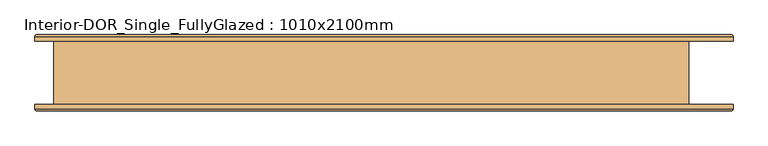
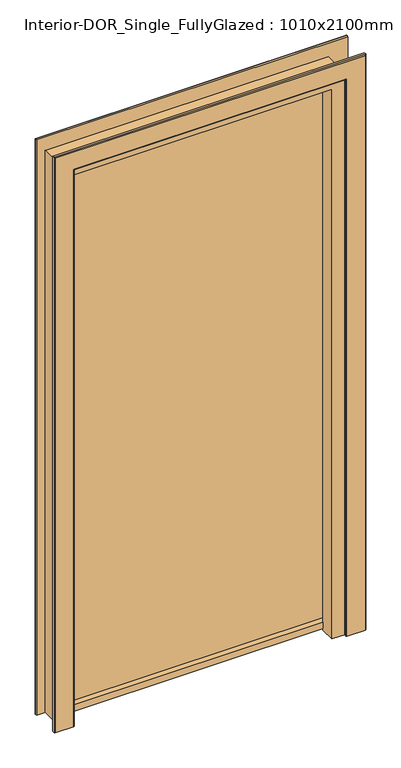
"""IFC4 building model written with IfcOpenShell, lengths in millimetres: door geometry, Interior-DOR_Single_FullyGlazed : 1010x2100mm."""

import ifcopenshell
import ifcopenshell.guid

model = None  # the IFC model being written
_history = None  # IfcOwnerHistory: only IFC2X3 demands one
_inside = {}  # id of a spatial element -> (the spatial element, [elements in it])
_under = {}  # id of a project, library or spatial element -> (it, [spatial elements below it])
_declared = {}  # id of a project -> (the project, [libraries it declares])
_typed = {}  # id of a type object -> (the type object, [elements of that type])
_made_of = {}  # id of a material, layer set ... -> (it, [elements and type objects made of it])


def new_model(schema):
    """Start an empty IFC model of exactly this schema.

    Asked for "IFC4X3", IfcOpenShell would pick the latest addendum, in which some entities
    have other attributes; the version numbers below select the first issue.
    IFC2X3 requires an IfcOwnerHistory on every rooted entity: one is made here for all.
    """
    global model, _history
    if schema == "IFC4X3":
        model = ifcopenshell.file(schema_version=(4, 3, 0, 0))
    else:
        model = ifcopenshell.file(schema=schema)
    _inside.clear()
    _under.clear()
    _declared.clear()
    _typed.clear()
    _made_of.clear()
    _history = None
    if model.schema == "IFC2X3":
        org = make("IfcOrganization", Name="unknown")
        user = make(
            "IfcPersonAndOrganization",
            ThePerson=make("IfcPerson", FamilyName="unknown"),
            TheOrganization=org,
        )
        app = make(
            "IfcApplication",
            ApplicationDeveloper=org,
            Version="unknown",
            ApplicationFullName="unknown",
            ApplicationIdentifier="unknown",
        )
        _history = make(
            "IfcOwnerHistory",
            OwningUser=user,
            OwningApplication=app,
            ChangeAction="ADDED",
            CreationDate=0,
        )
    return model


def make(cls, **values):
    """One entity of the class cls with the attributes given. An attribute that is None is left unset."""
    return model.create_entity(
        cls, **{name: value for name, value in values.items() if value is not None}
    )


def rooted(cls, **values):
    """An entity with a GlobalId (a new one), such as an element, a storey or a relation."""
    return make(cls, GlobalId=ifcopenshell.guid.new(), OwnerHistory=_history, **values)


def si_unit(unit_type, name, prefix=None):
    """IfcSIUnit, for example si_unit("LENGTHUNIT", "METRE", prefix="MILLI")."""
    return make("IfcSIUnit", UnitType=unit_type, Prefix=prefix, Name=name)


def assignment(units):
    """IfcUnitAssignment: the units of a project."""
    return None if units is None else make("IfcUnitAssignment", Units=units)


def point(xyz):
    """IfcCartesianPoint."""
    return None if xyz is None else make("IfcCartesianPoint", Coordinates=xyz)


def direction(xyz):
    """IfcDirection."""
    return None if xyz is None else make("IfcDirection", DirectionRatios=xyz)


def frame(location, z_axis=None, x_axis=None):
    """IfcAxis2Placement3D, a coordinate frame: its origin and axes. An axis left out is left unset."""
    return make(
        "IfcAxis2Placement3D",
        Location=point(location),
        Axis=direction(z_axis),
        RefDirection=direction(x_axis),
    )


def origin():
    """The frame at (0, 0, 0) with its axes left unset."""
    return frame((0.0, 0.0, 0.0))


def place(relative_to, where):
    """IfcLocalPlacement: puts the frame where relative to a parent placement (None: the world)."""
    return make(
        "IfcLocalPlacement", PlacementRelTo=relative_to, RelativePlacement=where
    )


def context(
    kind, dimensions, precision=None, world=None, true_north=None, identifier=None
):
    """IfcGeometricRepresentationContext, for example the 3D "Model" context."""
    return make(
        "IfcGeometricRepresentationContext",
        ContextIdentifier=identifier,
        ContextType=kind,
        CoordinateSpaceDimension=dimensions,
        Precision=precision,
        WorldCoordinateSystem=world,
        TrueNorth=true_north,
    )


def project(units=None, contexts=None):
    """IfcProject with its units and contexts."""
    return rooted(
        "IfcProject",
        Name="project",
        RepresentationContexts=contexts,
        UnitsInContext=assignment(units),
    )


def spatial(cls, under=None, at=None, **own):
    """A site, building, storey or space (cls), placed at a placement, below another one or the project."""
    s = rooted(cls, ObjectPlacement=at, **own)
    if under is not None:
        _under.setdefault(under.id(), (under, []))[1].append(s)
    return s


def polyline(points):
    """IfcPolyline through the points."""
    return make("IfcPolyline", Points=[point(p) for p in points])


def circle_curve(where, radius):
    """IfcCircle in the frame where."""
    return make("IfcCircle", Position=where, Radius=radius)


def ellipse_curve(where, semi_axis1, semi_axis2):
    """IfcEllipse in the frame where."""
    return make(
        "IfcEllipse", Position=where, SemiAxis1=semi_axis1, SemiAxis2=semi_axis2
    )


def outline(outer, holes=None, kind="AREA"):
    """IfcArbitraryClosedProfileDef: a profile drawn as a closed curve; with holes, ...WithVoids."""
    if holes is None:
        return make("IfcArbitraryClosedProfileDef", ProfileType=kind, OuterCurve=outer)
    return make(
        "IfcArbitraryProfileDefWithVoids",
        ProfileType=kind,
        OuterCurve=outer,
        InnerCurves=holes,
    )


def extrude(swept, where, along, depth):
    """IfcExtrudedAreaSolid: the profile swept, set in the frame where, extruded along a direction by depth."""
    return make(
        "IfcExtrudedAreaSolid",
        SweptArea=swept,
        Position=where,
        ExtrudedDirection=direction(along),
        Depth=depth,
    )


def faces_of(points, faces, orient=None, outer=None):
    """IfcFace entities. A face is a list of loops; a loop is a list of indices into points, from 0.

    orient and outer hold one flag for each loop. By default every Orientation is true, the
    first loop of a face is its IfcFaceOuterBound and the others are IfcFaceBound.
    """
    made = []
    for i, loops in enumerate(faces):
        bounds = []
        for j, loop in enumerate(loops):
            is_outer = j == 0 if outer is None else outer[i][j]
            bounds.append(
                make(
                    "IfcFaceOuterBound" if is_outer else "IfcFaceBound",
                    Bound=make("IfcPolyLoop", Polygon=[points[k] for k in loop]),
                    Orientation=True if orient is None else orient[i][j],
                )
            )
        made.append(make("IfcFace", Bounds=bounds))
    return made


def faceted_brep(points, faces, orient=None, outer=None, voids=None):
    """IfcFacetedBrep: a solid bounded by flat faces; with voids (closed shells), ...WithVoids."""
    shared = [point(p) for p in points]
    hull = make("IfcClosedShell", CfsFaces=faces_of(shared, faces, orient, outer))
    if voids is None:
        return make("IfcFacetedBrep", Outer=hull)
    return make(
        "IfcFacetedBrepWithVoids",
        Outer=hull,
        Voids=[
            make(cls, CfsFaces=faces_of(shared, fs, o, b)) for cls, fs, o, b in voids
        ],
    )


def shape(context_of_items, identifier, shape_type, items):
    """IfcShapeRepresentation: the items that make up one representation, for example the "Body"."""
    return make(
        "IfcShapeRepresentation",
        ContextOfItems=context_of_items,
        RepresentationIdentifier=identifier,
        RepresentationType=shape_type,
        Items=items,
    )


def source(mapping_origin, context_of_items, identifier, shape_type, items):
    """IfcRepresentationMap: a shape defined once, which mapped items show again and again."""
    return make(
        "IfcRepresentationMap",
        MappingOrigin=mapping_origin,
        MappedRepresentation=shape(context_of_items, identifier, shape_type, items),
    )


def transform(
    local_origin,
    x_axis=None,
    y_axis=None,
    z_axis=None,
    scale=None,
    scale2=None,
    scale3=None,
    uniform=True,
):
    """IfcCartesianTransformationOperator3D, or its non-uniform kind. x_axis, y_axis, z_axis: its Axis1, 2, 3."""
    if uniform:
        return make(
            "IfcCartesianTransformationOperator3D",
            Axis1=direction(x_axis),
            Axis2=direction(y_axis),
            LocalOrigin=point(local_origin),
            Scale=scale,
            Axis3=direction(z_axis),
        )
    return make(
        "IfcCartesianTransformationOperator3DnonUniform",
        Axis1=direction(x_axis),
        Axis2=direction(y_axis),
        LocalOrigin=point(local_origin),
        Scale=scale,
        Axis3=direction(z_axis),
        Scale2=scale2,
        Scale3=scale3,
    )


def mapped(mapping_source, mapping_target):
    """IfcMappedItem: shows the shape of a source again, moved by a transform."""
    return make(
        "IfcMappedItem", MappingSource=mapping_source, MappingTarget=mapping_target
    )


def made_of(thing, what):
    """Note that an element or type object is made of a material, layer set ...; save() writes the relation."""
    if what is not None:
        _made_of.setdefault(what.id(), (what, []))[1].append(thing)
    return thing


def element(
    cls,
    number,
    at=None,
    inside=None,
    cuts=None,
    type_object=None,
    material=None,
    context=None,
    identifier="Body",
    shape_type=None,
    held_by="IfcProductDefinitionShape",
    body=None,
    shapes=None,
    **own,
):
    """One element of the class cls, such as IfcWall. Its Tag is "e" and its number.

    at: its placement. inside: the storey or other place that contains it. cuts: it is an
    opening in that element (IfcRelVoidsElement). A single representation is given by context,
    identifier, shape_type and body (its items); several are given by shapes. held_by: the class
    of the entity that holds the representations. save() writes the other relations.
    """
    e = rooted(cls, Tag="e%d" % number, ObjectPlacement=at, **own)
    if body is not None:
        shapes = [shape(context, identifier, shape_type, body)]
    if shapes is not None:
        e.Representation = make(held_by, Representations=shapes)
    if inside is not None:
        _inside.setdefault(inside.id(), (inside, []))[1].append(e)
    if cuts is not None:
        rooted(
            "IfcRelVoidsElement", RelatingBuildingElement=cuts, RelatedOpeningElement=e
        )
    if type_object is not None:
        _typed.setdefault(type_object.id(), (type_object, []))[1].append(e)
    return made_of(e, material)


def aggregate(whole, parts):
    """IfcRelAggregates: a whole, such as a stair, and the parts it consists of."""
    return rooted("IfcRelAggregates", RelatingObject=whole, RelatedObjects=parts)


def save(model, path):
    """Write the relations noted so far, then the file.

    IfcRelAggregates (storeys below a building ...), IfcRelContainedInSpatialStructure (elements
    in a storey), IfcRelDefinesByType, IfcRelAssociatesMaterial and IfcRelDeclares: one each for
    every whole, place, type object, material and project.
    """
    for whole, parts in _under.values():
        aggregate(whole, parts)
    for where, things in _inside.values():
        rooted(
            "IfcRelContainedInSpatialStructure",
            RelatedElements=things,
            RelatingStructure=where,
        )
    for kind, things in _typed.values():
        rooted("IfcRelDefinesByType", RelatedObjects=things, RelatingType=kind)
    for what, things in _made_of.values():
        rooted("IfcRelAssociatesMaterial", RelatedObjects=things, RelatingMaterial=what)
    for by, libraries in _declared.values():
        rooted("IfcRelDeclares", RelatingContext=by, RelatedDefinitions=libraries)
    model.write(path)


def plane_surface(at):
    """IfcPlane: the flat surface through the origin of the frame at, square to its z axis."""
    return make("IfcPlane", Position=at)


def cylinder_surface(at, radius):
    """IfcCylindricalSurface: all points at the distance radius from the z axis of the frame at."""
    return make("IfcCylindricalSurface", Position=at, Radius=radius)


def advanced_brep(points, edges, surfaces, faces):
    """IfcAdvancedBrep: a solid bounded by faces that lie on surfaces and meet in shared edges.

    An edge is (start, end): straight between two places in points (the first is 0);
    or (start, end, curve); or (start, end, curve, False) where it runs against its curve.
    A face is (place in surfaces, loops), or (place, loops, False) where it looks against
    its surface's normal. A loop lists edges by number (the first is 1), with a minus sign
    where the edge is run from its end to its start. The first loop is the outer one.
    """
    corners = [point(p) for p in points]
    vertices = [make("IfcVertexPoint", VertexGeometry=c) for c in corners]
    made = []
    for start, end, *more in edges:
        made.append(
            make(
                "IfcEdgeCurve",
                EdgeStart=vertices[start],
                EdgeEnd=vertices[end],
                EdgeGeometry=more[0] if more else make("IfcPolyline", Points=[corners[start], corners[end]]),
                SameSense=more[1] if len(more) > 1 else True,
            )
        )
    hull = []
    for where, loops, *sense in faces:
        bounds = []
        for j, loop in enumerate(loops):
            ring = [make("IfcOrientedEdge", EdgeElement=made[abs(k) - 1], Orientation=k > 0) for k in loop]
            bounds.append(
                make(
                    "IfcFaceOuterBound" if j == 0 else "IfcFaceBound",
                    Bound=make("IfcEdgeLoop", EdgeList=ring),
                    Orientation=True,
                )
            )
        hull.append(make("IfcAdvancedFace", Bounds=bounds, FaceSurface=surfaces[where], SameSense=sense[0] if sense else True))
    return make("IfcAdvancedBrep", Outer=make("IfcClosedShell", CfsFaces=hull))


def interior_dor_single_fullyglazed_1010x2100mm_4e97d53e(model_context):
    return source(origin(), model_context, "Body", "SolidModel", [
        advanced_brep(
        [(-460.0, 50.0, 0.0), (-530.0, 50.0, 0.0), (-530.0, 57.0, 0.0), (-527.0, 60.0, 0.0), (-463.0, 60.0, 0.0), (-460.0, 57.0, 0.0), (-460.0, 57.0, 2075.0), (-460.0, 50.0, 2075.0), (-463.0, 60.0, 2078.0), (-527.0, 60.0, 2142.0), (567.0, 60.0, 2142.0), (567.0, 60.0, 0.0), (503.0, 60.0, 0.0), (503.0, 60.0, 2078.0), (-530.0, 57.0, 2145.0), (-530.0, 50.0, 2145.0), (500.0, 50.0, 2075.0), (500.0, 50.0, 0.0), (570.0, 50.0, 0.0), (570.0, 50.0, 2145.0), (500.0, 57.0, 0.0), (500.0, 57.0, 2075.0), (570.0, 57.0, 0.0), (570.0, 57.0, 2145.0)],
        [
            (0, 1),
            (1, 2),
            (2, 3, circle_curve(frame((-527.0, 57.0, 0.0), z_axis=(0.0, 0.0, -1.0), x_axis=(-1.0, 0.0, 0.0)), 3.0)),
            (3, 4),
            (4, 5, circle_curve(frame((-463.0, 57.0, 0.0), z_axis=(0.0, 0.0, -1.0), x_axis=(-1.0, 0.0, 0.0)), 3.0)),
            (5, 0),
            (5, 6),
            (6, 7),
            (7, 0),
            (4, 8),
            (8, 6, ellipse_curve(frame((-463.0, 57.0, 2078.0), z_axis=(-0.7071067811865475, 0.0, -0.7071067811865475), x_axis=(0.7071067811865474, 0.0, -0.7071067811865476)), 4.2426407, 3.0)),
            (3, 9),
            (9, 10),
            (10, 11),
            (11, 12),
            (12, 13),
            (13, 8),
            (2, 14),
            (14, 9, ellipse_curve(frame((-527.0, 57.0, 2142.0), z_axis=(-0.7071067811865475, 0.0, -0.7071067811865475), x_axis=(0.7071067811865474, 0.0, -0.7071067811865476)), 4.2426407, 3.0)),
            (1, 15),
            (15, 14),
            (7, 16),
            (16, 17),
            (17, 18),
            (18, 19),
            (19, 15),
            (12, 20, circle_curve(frame((503.0, 57.0, 0.0), z_axis=(0.0, 0.0, 1.0), x_axis=(1.0, 0.0, 0.0)), 3.0)),
            (20, 21),
            (21, 13, ellipse_curve(frame((503.0, 57.0, 2078.0), z_axis=(0.7071067811865475, 0.0, -0.7071067811865475), x_axis=(0.7071067811865474, 0.0, 0.7071067811865476)), 4.2426407, 3.0)),
            (17, 20),
            (11, 22, circle_curve(frame((567.0, 57.0, 0.0), z_axis=(0.0, 0.0, -1.0), x_axis=(1.0, 0.0, 0.0)), 3.0)),
            (22, 18),
            (23, 22),
            (10, 23, ellipse_curve(frame((567.0, 57.0, 2142.0), z_axis=(0.7071067811865475, 0.0, -0.7071067811865475), x_axis=(0.7071067811865474, 0.0, 0.7071067811865476)), 4.2426407, 3.0)),
            (23, 19),
            (16, 21),
            (6, 21),
            (14, 23),
        ],
        [
            plane_surface(frame((-480.0, -50.0, 0.0), z_axis=(0.0, 0.0, -1.0), x_axis=(0.0, 1.0, 0.0))),
            plane_surface(frame((-460.0, 50.0, 0.0), z_axis=(1.0, 0.0, 0.0), x_axis=(0.0, 0.0, 1.0))),
            cylinder_surface(frame((-463.0, 57.0, 0.0), z_axis=(0.0, 0.0, -1.0), x_axis=(-1.0, 0.0, 0.0)), 3.0),
            plane_surface(frame((-463.0, 60.0, 0.0), z_axis=(0.0, 1.0, 0.0), x_axis=(0.0, 0.0, 1.0))),
            cylinder_surface(frame((-527.0, 57.0, 0.0), z_axis=(0.0, 0.0, -1.0), x_axis=(-1.0, 0.0, 0.0)), 3.0),
            plane_surface(frame((-530.0, 57.0, 0.0), z_axis=(-1.0, 0.0, 0.0), x_axis=(0.0, 0.0, 1.0))),
            plane_surface(frame((-530.0, 50.0, 0.0), z_axis=(0.0, -1.0, 0.0), x_axis=(0.0, 0.0, 1.0))),
            cylinder_surface(frame((503.0, 57.0, 2095.0), z_axis=(0.0, 0.0, 1.0), x_axis=(1.0, 0.0, 0.0)), 3.0),
            plane_surface(frame((520.0, -50.0, 0.0), z_axis=(0.0, 0.0, -1.0), x_axis=(0.0, 1.0, 0.0))),
            cylinder_surface(frame((567.0, 57.0, 2095.0), z_axis=(0.0, 0.0, 1.0), x_axis=(1.0, 0.0, 0.0)), 3.0),
            plane_surface(frame((570.0, 57.0, 2145.0), z_axis=(1.0, 0.0, 0.0), x_axis=(0.0, 0.0, -1.0))),
            plane_surface(frame((500.0, 50.0, 2075.0), z_axis=(-1.0, 0.0, 0.0), x_axis=(0.0, 0.0, -1.0))),
            plane_surface(frame((-460.0, 50.0, 2075.0), z_axis=(0.0, 0.0, -1.0), x_axis=(1.0, 0.0, 0.0))),
            cylinder_surface(frame((-480.0, 57.0, 2078.0), z_axis=(-1.0, 0.0, 0.0), x_axis=(0.0, 0.0, 1.0)), 3.0),
            cylinder_surface(frame((-480.0, 57.0, 2142.0), z_axis=(-1.0, 0.0, 0.0), x_axis=(0.0, 0.0, 1.0)), 3.0),
            plane_surface(frame((-530.0, 57.0, 2145.0), z_axis=(0.0, 0.0, 1.0), x_axis=(1.0, 0.0, 0.0))),
        ],
        [
            (0, [[1, 2, 3, 4, 5, 6]]),
            (1, [[7, 8, 9, -6]]),
            (2, [[10, 11, -7, -5]]),
            (3, [[12, 13, 14, 15, 16, 17, -10, -4]]),
            (4, [[18, 19, -12, -3]]),
            (5, [[20, 21, -18, -2]]),
            (6, [[-9, 22, 23, 24, 25, 26, -20, -1]]),
            (7, [[-16, 27, 28, 29]]),
            (8, [[30, -27, -15, 31, 32, -24]]),
            (9, [[33, -31, -14, 34]]),
            (10, [[-25, -32, -33, 35]]),
            (11, [[-28, -30, -23, 36]]),
            (12, [[37, -36, -22, -8]]),
            (13, [[-17, -29, -37, -11]]),
            (14, [[38, -34, -13, -19]]),
            (15, [[-26, -35, -38, -21]]),
        ],
    ),
        advanced_brep(
        [(-530.0, -50.0, 0.0), (-460.0, -50.0, 0.0), (-460.0, -57.0, 0.0), (-463.0, -60.0, 0.0), (-527.0, -60.0, 0.0), (-530.0, -57.0, 0.0), (-530.0, -57.0, 2145.0), (-530.0, -50.0, 2145.0), (-527.0, -60.0, 2142.0), (-463.0, -60.0, 2078.0), (503.0, -60.0, 2078.0), (503.0, -60.0, 0.0), (567.0, -60.0, 0.0), (567.0, -60.0, 2142.0), (-460.0, -57.0, 2075.0), (-460.0, -50.0, 2075.0), (570.0, -50.0, 2145.0), (570.0, -50.0, 0.0), (500.0, -50.0, 0.0), (500.0, -50.0, 2075.0), (570.0, -57.0, 0.0), (570.0, -57.0, 2145.0), (500.0, -57.0, 0.0), (500.0, -57.0, 2075.0)],
        [
            (0, 1),
            (1, 2),
            (2, 3, circle_curve(frame((-463.0, -57.0, 0.0), z_axis=(0.0, 0.0, -1.0), x_axis=(-1.0, 0.0, 0.0)), 3.0)),
            (3, 4),
            (4, 5, circle_curve(frame((-527.0, -57.0, 0.0), z_axis=(0.0, 0.0, -1.0), x_axis=(-1.0, 0.0, 0.0)), 3.0)),
            (5, 0),
            (5, 6),
            (6, 7),
            (7, 0),
            (4, 8),
            (8, 6, ellipse_curve(frame((-527.0, -57.0, 2142.0), z_axis=(-0.7071067811865475, 0.0, -0.7071067811865475), x_axis=(0.7071067811865474, 0.0, -0.7071067811865476)), 4.2426407, 3.0)),
            (3, 9),
            (9, 10),
            (10, 11),
            (11, 12),
            (12, 13),
            (13, 8),
            (2, 14),
            (14, 9, ellipse_curve(frame((-463.0, -57.0, 2078.0), z_axis=(-0.7071067811865475, 0.0, -0.7071067811865475), x_axis=(0.7071067811865474, 0.0, -0.7071067811865476)), 4.2426407, 3.0)),
            (1, 15),
            (15, 14),
            (7, 16),
            (16, 17),
            (17, 18),
            (18, 19),
            (19, 15),
            (12, 20, circle_curve(frame((567.0, -57.0, 0.0), z_axis=(0.0, 0.0, 1.0), x_axis=(1.0, 0.0, 0.0)), 3.0)),
            (20, 21),
            (21, 13, ellipse_curve(frame((567.0, -57.0, 2142.0), z_axis=(0.7071067811865475, 0.0, -0.7071067811865475), x_axis=(0.7071067811865474, 0.0, 0.7071067811865476)), 4.2426407, 3.0)),
            (17, 20),
            (11, 22, circle_curve(frame((503.0, -57.0, 0.0), z_axis=(0.0, 0.0, -1.0), x_axis=(1.0, 0.0, 0.0)), 3.0)),
            (22, 18),
            (23, 22),
            (10, 23, ellipse_curve(frame((503.0, -57.0, 2078.0), z_axis=(0.7071067811865475, 0.0, -0.7071067811865475), x_axis=(0.7071067811865474, 0.0, 0.7071067811865476)), 4.2426407, 3.0)),
            (23, 19),
            (16, 21),
            (6, 21),
            (14, 23),
        ],
        [
            plane_surface(frame((-480.0, -50.0, 0.0), z_axis=(0.0, 0.0, -1.0), x_axis=(0.0, 1.0, 0.0))),
            plane_surface(frame((-530.0, -50.0, 0.0), z_axis=(-1.0, 0.0, 0.0), x_axis=(0.0, 0.0, 1.0))),
            cylinder_surface(frame((-527.0, -57.0, 0.0), z_axis=(0.0, 0.0, -1.0), x_axis=(-1.0, 0.0, 0.0)), 3.0),
            plane_surface(frame((-527.0, -60.0, 0.0), z_axis=(0.0, -1.0, 0.0), x_axis=(0.0, 0.0, 1.0))),
            cylinder_surface(frame((-463.0, -57.0, 0.0), z_axis=(0.0, 0.0, -1.0), x_axis=(-1.0, 0.0, 0.0)), 3.0),
            plane_surface(frame((-460.0, -57.0, 0.0), z_axis=(1.0, 0.0, 0.0), x_axis=(0.0, 0.0, 1.0))),
            plane_surface(frame((-460.0, -50.0, 0.0), z_axis=(0.0, 1.0, 0.0), x_axis=(0.0, 0.0, 1.0))),
            cylinder_surface(frame((567.0, -57.0, 2095.0), z_axis=(0.0, 0.0, 1.0), x_axis=(1.0, 0.0, 0.0)), 3.0),
            plane_surface(frame((520.0, -50.0, 0.0), z_axis=(0.0, 0.0, -1.0), x_axis=(0.0, 1.0, 0.0))),
            cylinder_surface(frame((503.0, -57.0, 2095.0), z_axis=(0.0, 0.0, 1.0), x_axis=(1.0, 0.0, 0.0)), 3.0),
            plane_surface(frame((500.0, -57.0, 2075.0), z_axis=(-1.0, 0.0, 0.0), x_axis=(0.0, 0.0, -1.0))),
            plane_surface(frame((570.0, -50.0, 2145.0), z_axis=(1.0, 0.0, 0.0), x_axis=(0.0, 0.0, -1.0))),
            plane_surface(frame((-530.0, -50.0, 2145.0), z_axis=(0.0, 0.0, 1.0), x_axis=(1.0, 0.0, 0.0))),
            cylinder_surface(frame((-480.0, -57.0, 2142.0), z_axis=(-1.0, 0.0, 0.0), x_axis=(0.0, 0.0, 1.0)), 3.0),
            cylinder_surface(frame((-480.0, -57.0, 2078.0), z_axis=(-1.0, 0.0, 0.0), x_axis=(0.0, 0.0, 1.0)), 3.0),
            plane_surface(frame((-460.0, -57.0, 2075.0), z_axis=(0.0, 0.0, -1.0), x_axis=(1.0, 0.0, 0.0))),
        ],
        [
            (0, [[1, 2, 3, 4, 5, 6]]),
            (1, [[7, 8, 9, -6]]),
            (2, [[10, 11, -7, -5]]),
            (3, [[12, 13, 14, 15, 16, 17, -10, -4]]),
            (4, [[18, 19, -12, -3]]),
            (5, [[20, 21, -18, -2]]),
            (6, [[-9, 22, 23, 24, 25, 26, -20, -1]]),
            (7, [[-16, 27, 28, 29]]),
            (8, [[30, -27, -15, 31, 32, -24]]),
            (9, [[33, -31, -14, 34]]),
            (10, [[-25, -32, -33, 35]]),
            (11, [[-28, -30, -23, 36]]),
            (12, [[37, -36, -22, -8]]),
            (13, [[-17, -29, -37, -11]]),
            (14, [[38, -34, -13, -19]]),
            (15, [[-26, -35, -38, -21]]),
        ],
    ),
        extrude(outline(polyline([(470.0, 31.0), (470.0, 24.0), (-430.0, 24.0), (-430.0, 31.0), (470.0, 31.0)])), frame((0.0, 0.0, 30.0), z_axis=(0.0, 0.0, 1.0), x_axis=(1.0, 0.0, 0.0)), (0.0, 0.0, 1.0), 2015.0),
        extrude(outline(polyline([(5.0, -455.0), (5.0, 495.0), (2070.0, 495.0), (2070.0, -455.0), (5.0, -455.0)]), holes=[polyline([(2045.0, 470.0), (30.0, 470.0), (30.0, -430.0), (2045.0, -430.0), (2045.0, 470.0)])]), frame((0.0, 5.0, 0.0), z_axis=(0.0, 1.0, 0.0), x_axis=(0.0, 0.0, 1.0)), (0.0, 0.0, 1.0), 45.0),
        faceted_brep([(-500.0, -50.0, 0.0), (-500.0, 50.0, 0.0), (-475.0, 50.0, 0.0), (-475.0, 5.0, 0.0), (-455.0, 5.0, 0.0), (-455.0, -50.0, 0.0), (-455.0, -50.0, 2050.0), (455.0, -50.0, 2050.0), (455.0, -50.0, 0.0), (500.0, -50.0, 0.0), (500.0, -50.0, 2095.0), (-500.0, -50.0, 2095.0), (-455.0, 5.0, 2050.0), (-475.0, 5.0, 2070.0), (475.0, 5.0, 2070.0), (475.0, 5.0, 0.0), (455.0, 5.0, 0.0), (455.0, 5.0, 2050.0), (-475.0, 50.0, 2070.0), (-500.0, 50.0, 2095.0), (500.0, 50.0, 2095.0), (500.0, 50.0, 0.0), (475.0, 50.0, 0.0), (475.0, 50.0, 2070.0)], [[[0, 1, 2, 3, 4, 5]], [[5, 6, 7, 8, 9, 10, 11, 0]], [[4, 12, 6, 5]], [[3, 13, 14, 15, 16, 17, 12, 4]], [[2, 18, 13, 3]], [[1, 19, 20, 21, 22, 23, 18, 2]], [[0, 11, 19, 1]], [[10, 9, 21, 20]], [[9, 8, 16, 15, 22, 21]], [[17, 16, 8, 7]], [[23, 22, 15, 14]], [[12, 17, 7, 6]], [[18, 23, 14, 13]], [[11, 10, 20, 19]]]),
    ])


if __name__ == "__main__":
    model = new_model("IFC4")
    model_context = context("Model", 3, world=origin())
    ifc_project = project(units=[si_unit("LENGTHUNIT", "METRE", prefix="MILLI")], contexts=[model_context])
    site = spatial("IfcSite", under=ifc_project)
    building = spatial("IfcBuilding", under=site)
    placement = place(None, origin())
    interior_dor_single_fullyglazed_1010x2100mm_shape = interior_dor_single_fullyglazed_1010x2100mm_4e97d53e(model_context)
    element("IfcDoor", 1, ObjectType="Interior-DOR_Single_FullyGlazed : 1010x2100mm", at=placement, inside=building, context=model_context, shape_type="MappedRepresentation", body=[
        mapped(interior_dor_single_fullyglazed_1010x2100mm_shape, transform((0.0, 0.0, 0.0), x_axis=(1.0, 0.0, 0.0), y_axis=(0.0, 1.0, 0.0), z_axis=(0.0, 0.0, 1.0))),
    ])
    save(model, "model.ifc")

# Revit data of these elements
# Type "Interior-DOR_Single_FullyGlazed : 1010x2100mm"
#   Type IfcGUID = "2NKTNbJKP36hSTtB23u7pq"
#   Type Mark = "187"
#   Classification.Uniclass.EF.Number = "EF_25_30"
#   Classification.Uniclass.EF.Description = "Doors and windows"
#   WindLoadRating = "n/a"
#   WaterTightnessRating = "n/a"
#   WarrantyStartDate [instance default] = "1900-12-31T23:59:59"
#   WarrantyGuarantorParts = "n/a"
#   WarrantyGuarantorLabor = "n/a"
#   WarrantyDurationUnit = "year"
#   WarrantyDurationParts = "n/a"
#   WarrantyDurationLabor = "n/a"
#   WarrantyDescription = "n/a"
#   Version = "2"
#   Uniclass2015Version = "Systems v1.9"
#   Uniclass2015Title = "Doorset systems"
#   Uniclass2015Code = "Ss_25_30_20_25"
#   URL = "www.nationalbimlibrary.com"
#   TagNumber [instance default] = "n/a"
#   SustainabilityPerformance = "n/a"
#   Status = "UNSET"
#   Size = "1010 x 2100 mm"
#   Shape = "n/a"
#   SerialNumber [instance default] = "n/a"
#   SecurityRating = "n/a"
#   Revision = "n/a"
#   ReplacementCost = "n/a"
#   Reference = "n/a"
#   ProductInformation = "n/a"
#   Operation = "SINGLE_SWING_RIGHT"
#   OmniClassVersion = "Table 22 2012-05-16"
#   OmniClassTitle = "Doors and Frames"
#   OmniClassCode = "22-08 10 00"
#   Name = "DoorsetSystem_Interior-Single_FullyGlazed"
#   NBSReference = "25-50-20/120"
#   NBSDescription = "Doorset system"
#   NBSCertification = "www.nationalbimlibrary.com/cert/43bi5322"
#   ModelReference = "Interior Single Door Fully Glazed Leaf"
#   ModelNumber = "n/a"
#   Model = "Interior Single Door Fully Glazed Leaf"
#   MechanicalLoadRating = "n/a"
#   Material = "n/a"
#   ManufacturerURL = "n/a"
#   ManufacturerName = "n/a"
#   Manufacturer = "info@theNBS.com"
#   InstallationDate [instance default] = "1900-12-31T23:59:59"
#   IfcExportType = "DOOR"
#   IfcExportAs = "IfcDoorType"
#   HygrothermalRating = "n/a"
#   Grade = "n/a"
#   GlassColor = "n/a"
#   FireRating = "n/a"
#   Fire Rating = "n/a"
#   Finish = "n/a"
#   FillGas = "n/a"
#   Features = "n/a"
#   ExpectedLife = "n/a"
#   DurationUnit = "n/a"
#   DurabilityRating = "n/a"
#   DoorNumber [instance default] = "n/a"
#   Description = "Generic single interior door with fully glazed leaf"
#   Construction Type = "USERDEFINED"
#   Constituents = "n/a"
#   ComponentNumber [instance default] = "n/a"
#   Color = "n/a"
#   CodePerformance = "n/a"
#   Category = "Ss_25_30_20_25:Doorset systems"
#   BarCode [instance default] = "n/a"
#   BIMObjectName = "NBS_DoorsetSystem_Interior-Single_FullyGlazed"
#   Author = "NBS"
#   AssetType = "Fixed"
#   AssetIdentifier [instance default] = "n/a"
#   AcousticRating = "n/a"
#   AccessibilityPerformance = "n/a"
#   WallThickness [instance default] = 0.15 m
#   VisibleLightTransmittance = 0
#   VisibileLightReflectance = 0
#   ThresholdHeight = 0.015 m
#   ThermalTransmittanceWinter = 0
#   ThermalTransmittanceSummer = 0
#   ThermalTransmittance = 0
#   StructuralToleranceJamb = 0.005 m
#   StructuralToleranceHead = 0.005 m
#   StructuralOpeningWidth = 1.01 m
#   StructuralOpeningHeight = 2.1 m
#   StructuralOpeningCutBeyondFaceInternalMinimum [instance default] = 0.005 m
#   StructuralOpeningCutBeyondFaceInternal [instance default] = 0.005 m
#   StructuralOpeningCutBeyondFaceExternal [instance default] = 0.005 m
#   StopProjection = 0.02 m
#   StopDepth = 0.04 m
#   SolarTransmittance = 0
#   SolarReflectance = 0
#   SolarHeatGainTransmittance = 0
#   SolarAbsorption = 0
#   ShadingCoefficient = 0
#   RebateDepth = 0.045 m
#   PanelWidth = 0.95 m
#   PanelHeight = 2.07 m
#   PanelDepth = 0.045 m
#   OpeningTolerance = 0 m
#   NominalWidth = 1.01 m
#   NominalLength = 0 m
#   NominalHeight = 2.1 m
#   PanelUndercut = 0.005 m
#   LayerWrapExternal [instance default] = 0.005 m
#   Infiltration = 0
#   GlazingPanelThickness = 0.007 m
#   GlazingCavityThicknessOuter = 0 m
#   GlazingCavityThicknessIntermediate = 0 m
#   GlazingCavityThicknessInner = 0 m
#   GlazingAreaFraction = 0
#   GlassThickness3 = 0.002 m
#   GlassThickness2 = 0.002 m
#   GlassThickness1 = 0.002 m
#   FrameThickness = 0.025 m
#   FrameSetback [instance default] = 0 m
#   FrameDepth [instance default] = 0.15 m
#   Height = 2.1 m
#   Width = 1.01 m
#   FinishThicknessInternal [instance default] = 0 m
#   FinishThicknessExternal [instance default] = 0 m
#   ClearOpeningWidth = 0.91 m
#   ClearOpeningHeight = 2.05 m
#   ArchitraveWidth = 0.07 m
#   ArchitraveThickness = 0.01 m
#   ArchitraveSetbackFromFrameFace = 0.005 m
#   SmokeStop = no
#   SingleRebate = yes
#   SelfClosing = no
#   PlantedStop = no
#   IsWired = no
#   IsTempered = no
#   IsLaminated = no
#   IsExternal = no
#   IsCoated = no
#   HasDrive = no
#   HandicapAccessible = no
#   GlazingUnitTriple = yes
#   GlazingUnitDouble = no
#   GlassLayers = 3
#   Wall Closure = 4
#   FireExit = no
#   PanelMaterial = NBS_Concept
#   GlazingPanelMaterial = NBS_Glass_Single
#   GlazingBeadMaterial = NBS_Concept
#   FrameSectionMaterial = NBS_Concept
#   Function = (empty or 0)
#   Cost = 0
# Element 1 (IfcDoor, "Interior-DOR_Single_FullyGlazed : 1010x2100mm")
#   WallThickness = 0.1 m
#   FrameDepth = 0.1 m
#   Materials on its faces: "NBS_Concept", "NBS_Glass_Single"
# Materials
#   "NBS_Concept": class "Generic", colour RGB 255 255 255, transparency 0, Description = "To be specified", Cost = 0
#   "NBS_Glass_Single": class "Glass", colour RGB 94 140 251, transparency 0.6, Cost = 0
